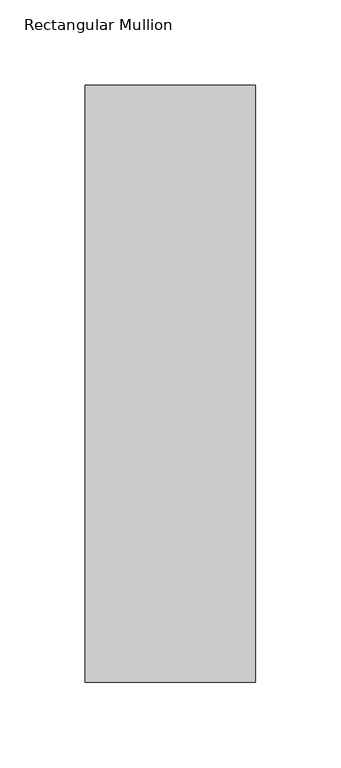
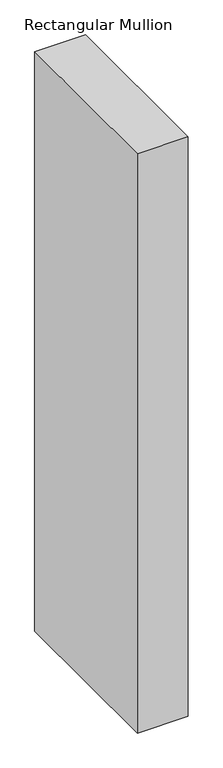
"""IFC4 building model written with IfcOpenShell, lengths in millimetres: member geometry, Rectangular Mullion : WWm-100x350-100mmOffset."""

from ifc_helpers import new_model, si_unit, frame, origin, place, context, project, spatial, polyline, outline, extrude, source, transform, mapped, element, save


def rectangular_mullion_3b5d59d4(model_context):
    return source(origin(), model_context, "Body", "SweptSolid", [
        extrude(outline(polyline([(0.0, 175.0), (0.0, -175.0), (-100.0, -175.0), (-100.0, 175.0), (0.0, 175.0)])), frame((0.0, 0.0, -1205.0), z_axis=(0.0, 0.0, 1.0), x_axis=(1.0, 0.0, 0.0)), (0.0, 0.0, 1.0), 1205.0),
    ])


if __name__ == "__main__":
    model = new_model("IFC4")
    model_context = context("Model", 3, world=origin())
    ifc_project = project(units=[si_unit("LENGTHUNIT", "METRE", prefix="MILLI")], contexts=[model_context])
    site = spatial("IfcSite", under=ifc_project)
    building = spatial("IfcBuilding", under=site)
    placement = place(None, origin())
    rectangular_mullion_shape = rectangular_mullion_3b5d59d4(model_context)
    element("IfcMember", 1, ObjectType="Rectangular Mullion : WWm-100x350-100mmOffset", at=placement, inside=building, context=model_context, shape_type="MappedRepresentation", body=[
        mapped(rectangular_mullion_shape, transform((0.0, 0.0, 0.0), x_axis=(1.0, 0.0, 0.0), y_axis=(0.0, 1.0, 0.0), z_axis=(0.0, 0.0, 1.0))),
    ])
    save(model, "model.ifc")

# Revit data of these elements
# Type "Rectangular Mullion : WWm-100x350-100mmOffset"
#   built-in parameter 1007304 = 1.14829 (stored number, unit not read)
#   built-in parameter 1007301 = 0.164042 (stored number, unit not read)
#   built-in parameter 1007300 = 0.164042 (stored number, unit not read)
# Element 1 (IfcMember, "Rectangular Mullion : WWm-100x350-100mmOffset")
#   Materials on its faces: "WW-EC-RGB-Mullion"
# Materials
#   "WW-EC-RGB-Mullion": class "Generic", colour RGB 255 255 255, transparency 0, Comments = "If region requests black mullions, switch asset color to RGB 25-25-25", Description = "Generic Color", Cost = 0
